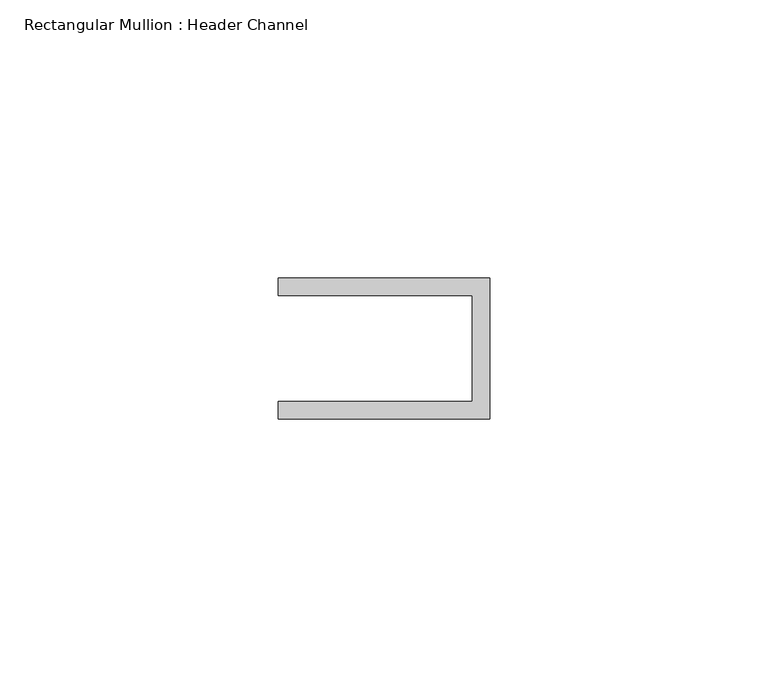
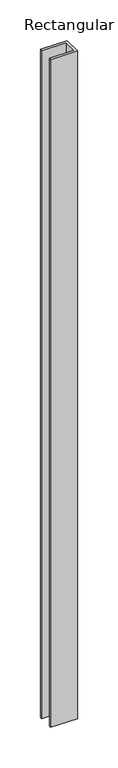
"""IFC4 building model written with IfcOpenShell, lengths in millimetres: member geometry, Rectangular Mullion : Header Channel."""

from ifc_helpers import new_model, si_unit, frame, origin, place, context, project, spatial, polyline, outline, extrude, source, transform, mapped, element, save


def rectangular_mullion_header_channel_9847aa58(model_context):
    return source(origin(), model_context, "Body", "SweptSolid", [
        extrude(outline(polyline([(0.0, -12.7), (-38.1, -12.7), (-38.1, -9.525), (-3.175, -9.525), (-3.175, 9.525), (-38.1, 9.525), (-38.1, 12.7), (0.0, 12.7), (0.0, -12.7)])), frame((0.0, 0.0, -1005.4166667), z_axis=(0.0, 0.0, 1.0), x_axis=(1.0, 0.0, 0.0)), (0.0, 0.0, 1.0), 1005.4166667),
    ])


if __name__ == "__main__":
    model = new_model("IFC4")
    model_context = context("Model", 3, world=origin())
    ifc_project = project(units=[si_unit("LENGTHUNIT", "METRE", prefix="MILLI")], contexts=[model_context])
    site = spatial("IfcSite", under=ifc_project)
    building = spatial("IfcBuilding", under=site)
    placement = place(None, origin())
    rectangular_mullion_header_channel_shape = rectangular_mullion_header_channel_9847aa58(model_context)
    element("IfcMember", 1, ObjectType="Rectangular Mullion : Header Channel", at=placement, inside=building, context=model_context, shape_type="MappedRepresentation", body=[
        mapped(rectangular_mullion_header_channel_shape, transform((0.0, 0.0, 0.0), x_axis=(1.0, 0.0, 0.0), y_axis=(0.0, 1.0, 0.0), z_axis=(0.0, 0.0, 1.0))),
    ])
    save(model, "model.ifc")

# Revit data of these elements
# Type "Rectangular Mullion : Header Channel"
#   built-in parameter 1007322 = 0.0833333 (stored number, unit not read)
#   built-in parameter 1007321 = -0.03125 (stored number, unit not read)
#   built-in parameter 1007320 = 0.0416667 (stored number, unit not read)
# Element 1 (IfcMember, "Rectangular Mullion : Header Channel")
#   Materials on its faces: "ALUM"
# Materials
#   "ALUM": class "Generic", colour RGB 157 157 157, transparency 0, Cost = 0
